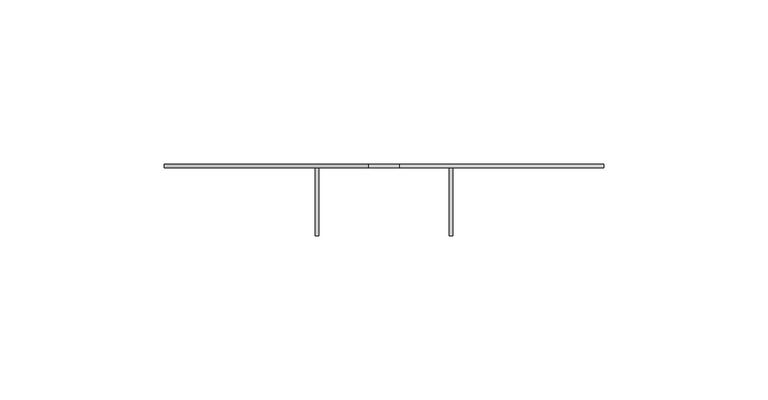
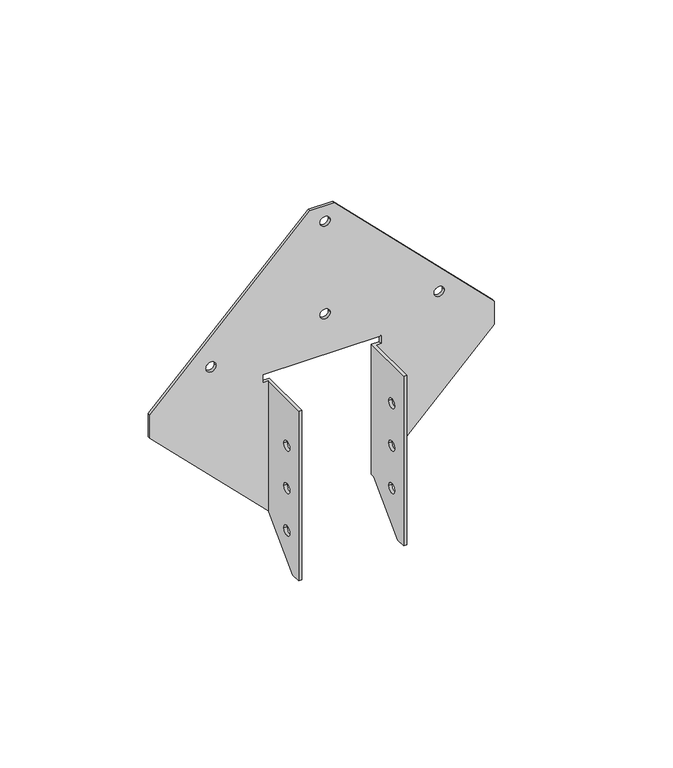
"""IFC4 building model written with IfcOpenShell, lengths in millimetres: proxy geometry, Simpson Strong-Tie H1 : Simpson Strong-Tie H1."""

from ifc_helpers import new_model, si_unit, frame, origin, place, context, project, spatial, polyline, circle_curve, source, transform, mapped, element, save
from ifc_brep_helpers import plane_surface, revolved_surface, advanced_brep


def generic_models_ac6e08b7(model_context):
    return source(origin(), model_context, "Body", "AdvancedBrep", [
        advanced_brep(
        [(-0.790575, 0.0, 54.76875), (-0.790575, -1.18872, 54.76875), (3.171825, -1.18872, 54.76875), (3.171825, 0.0, 54.76875), (-0.790575, 0.0, 16.66875), (-0.790575, -1.18872, 16.66875), (3.171825, -1.18872, 16.66875), (3.171825, 0.0, 16.66875), (43.659425, 0.0, 10.31875), (43.659425, -1.18872, 10.31875), (47.621825, -1.18872, 10.31875), (47.621825, 0.0, 10.31875), (-45.240575, 0.0, 10.31875), (-45.240575, -1.18872, 10.31875), (-41.278175, -1.18872, 10.31875), (-41.278175, 0.0, 10.31875), (19.84756, -11.902103, -19.05), (21.03628, -11.902103, -19.05), (21.03628, -15.864503, -19.05), (19.84756, -15.864503, -19.05), (19.84756, -11.902103, -36.5125), (21.03628, -11.902103, -36.5125), (21.03628, -15.864503, -36.5125), (19.84756, -15.864503, -36.5125), (19.84756, -11.902103, -53.975), (21.03628, -11.902103, -53.975), (21.03628, -15.864503, -53.975), (19.84756, -15.864503, -53.975), (-21.03628, -11.902103, -57.15), (-19.84756, -11.902103, -57.15), (-19.84756, -15.864503, -57.15), (-21.03628, -15.864503, -57.15), (-21.03628, -11.902103, -39.6875), (-19.84756, -11.902103, -39.6875), (-19.84756, -15.864503, -39.6875), (-21.03628, -15.864503, -39.6875), (-21.03628, -11.902103, -22.225), (-19.84756, -11.902103, -22.225), (-19.84756, -15.864503, -22.225), (-21.03628, -15.864503, -22.225), (23.08225, 0.0, 0.0), (23.08225, 0.0, -3.175), (23.08225, -1.18872, -3.175), (23.08225, -1.18872, 0.0), (21.03628, 0.0, -56.758894), (21.03628, -1.18872, -56.758894), (21.03628, -1.698923, -56.758894), (19.84756, -1.698923, -56.758894), (19.84756, 0.0, -56.758894), (19.84756, 0.0, -3.175), (19.84756, -21.820803, -3.175), (21.03628, -21.820803, -3.175), (21.03628, -1.18872, -3.175), (-23.08225, -1.18872, 0.0), (67.071875, -1.18872, -10.723299), (67.071875, -1.18872, -1.182951), (4.770174, -1.18872, 61.11875), (-4.770174, -1.18872, 61.11875), (-67.071875, -1.18872, -1.182951), (-67.071875, -1.18872, -10.723299), (-21.03628, -1.18872, -56.758894), (-21.03628, -1.18872, -3.175), (-23.08225, -1.18872, -3.175), (19.84756, -17.965029, -73.025), (19.84756, -21.820803, -73.025), (-21.03628, 0.0, -56.758894), (-19.84756, 0.0, -56.758894), (-19.84756, -1.698923, -56.758894), (-21.03628, -1.698923, -56.758894), (-23.08225, 0.0, 0.0), (-23.08225, 0.0, -3.175), (-19.84756, 0.0, -3.175), (-67.071875, 0.0, -10.723299), (-67.071875, 0.0, -1.182951), (-4.770174, 0.0, 61.11875), (4.770174, 0.0, 61.11875), (67.071875, 0.0, -1.182951), (67.071875, 0.0, -10.723299), (-21.03628, -21.820803, -3.175), (-19.84756, -21.820803, -3.175), (21.03628, -17.965029, -73.025), (21.03628, -21.820803, -73.025), (-19.84756, -21.820803, -73.025), (-19.84756, -17.965029, -73.025), (-21.03628, -17.965029, -73.025), (-21.03628, -21.820803, -73.025)],
        [
            (0, 1),
            (1, 2, circle_curve(frame((1.190625, -1.18872, 54.76875), z_axis=(0.0, -1.0, 0.0), x_axis=(-1.0, 0.0, 0.0)), 1.9812)),
            (2, 3),
            (3, 0, circle_curve(frame((1.190625, 0.0, 54.76875), z_axis=(0.0, 1.0, 0.0), x_axis=(-1.0, 0.0, 0.0)), 1.9812)),
            (4, 5),
            (5, 6, circle_curve(frame((1.190625, -1.18872, 16.66875), z_axis=(0.0, -1.0, 0.0), x_axis=(-1.0, 0.0, 0.0)), 1.9812)),
            (6, 7),
            (7, 4, circle_curve(frame((1.190625, 0.0, 16.66875), z_axis=(0.0, 1.0, 0.0), x_axis=(-1.0, 0.0, 0.0)), 1.9812)),
            (8, 9),
            (9, 10, circle_curve(frame((45.640625, -1.18872, 10.31875), z_axis=(0.0, -1.0, 0.0), x_axis=(-1.0, 0.0, 0.0)), 1.9812)),
            (10, 11),
            (11, 8, circle_curve(frame((45.640625, 0.0, 10.31875), z_axis=(0.0, 1.0, 0.0), x_axis=(-1.0, 0.0, 0.0)), 1.9812)),
            (12, 13),
            (13, 14, circle_curve(frame((-43.259375, -1.18872, 10.31875), z_axis=(0.0, -1.0, 0.0), x_axis=(-1.0, 0.0, 0.0)), 1.9812)),
            (14, 15),
            (15, 12, circle_curve(frame((-43.259375, 0.0, 10.31875), z_axis=(0.0, 1.0, 0.0), x_axis=(-1.0, 0.0, 0.0)), 1.9812)),
            (16, 17),
            (17, 18, circle_curve(frame((21.03628, -13.883303, -19.05), z_axis=(1.0, 0.0, 0.0), x_axis=(0.0, 1.0, 0.0)), 1.9812)),
            (18, 19),
            (19, 16, circle_curve(frame((19.84756, -13.883303, -19.05), z_axis=(-1.0, 0.0, 0.0), x_axis=(0.0, 1.0, 0.0)), 1.9812)),
            (20, 21),
            (21, 22, circle_curve(frame((21.03628, -13.883303, -36.5125), z_axis=(1.0, 0.0, 0.0), x_axis=(0.0, 1.0, 0.0)), 1.9812)),
            (22, 23),
            (23, 20, circle_curve(frame((19.84756, -13.883303, -36.5125), z_axis=(-1.0, 0.0, 0.0), x_axis=(0.0, 1.0, 0.0)), 1.9812)),
            (24, 25),
            (25, 26, circle_curve(frame((21.03628, -13.883303, -53.975), z_axis=(1.0, 0.0, 0.0), x_axis=(0.0, 1.0, 0.0)), 1.9812)),
            (26, 27),
            (27, 24, circle_curve(frame((19.84756, -13.883303, -53.975), z_axis=(-1.0, 0.0, 0.0), x_axis=(0.0, 1.0, 0.0)), 1.9812)),
            (28, 29),
            (29, 30, circle_curve(frame((-19.84756, -13.883303, -57.15), z_axis=(1.0, 0.0, 0.0), x_axis=(0.0, 1.0, 0.0)), 1.9812)),
            (30, 31),
            (31, 28, circle_curve(frame((-21.03628, -13.883303, -57.15), z_axis=(-1.0, 0.0, 0.0), x_axis=(0.0, 1.0, 0.0)), 1.9812)),
            (32, 33),
            (33, 34, circle_curve(frame((-19.84756, -13.883303, -39.6875), z_axis=(1.0, 0.0, 0.0), x_axis=(0.0, 1.0, 0.0)), 1.9812)),
            (34, 35),
            (35, 32, circle_curve(frame((-21.03628, -13.883303, -39.6875), z_axis=(-1.0, 0.0, 0.0), x_axis=(0.0, 1.0, 0.0)), 1.9812)),
            (36, 37),
            (37, 38, circle_curve(frame((-19.84756, -13.883303, -22.225), z_axis=(1.0, 0.0, 0.0), x_axis=(0.0, 1.0, 0.0)), 1.9812)),
            (38, 39),
            (39, 36, circle_curve(frame((-21.03628, -13.883303, -22.225), z_axis=(-1.0, 0.0, 0.0), x_axis=(0.0, 1.0, 0.0)), 1.9812)),
            (40, 41),
            (41, 42),
            (42, 43),
            (43, 40),
            (44, 45),
            (45, 46),
            (46, 47),
            (47, 48),
            (48, 44),
            (49, 50),
            (50, 51),
            (51, 52),
            (52, 42),
            (41, 49),
            (53, 43),
            (52, 45),
            (45, 54),
            (54, 55),
            (55, 56),
            (56, 57),
            (57, 58),
            (58, 59),
            (59, 60),
            (60, 61),
            (61, 62),
            (62, 53),
            (1, 2, circle_curve(frame((1.190625, -1.18872, 54.76875), z_axis=(0.0, 1.0, 0.0), x_axis=(-1.0, 0.0, 0.0)), 1.9812)),
            (5, 6, circle_curve(frame((1.190625, -1.18872, 16.66875), z_axis=(0.0, 1.0, 0.0), x_axis=(-1.0, 0.0, 0.0)), 1.9812)),
            (9, 10, circle_curve(frame((45.640625, -1.18872, 10.31875), z_axis=(0.0, 1.0, 0.0), x_axis=(-1.0, 0.0, 0.0)), 1.9812)),
            (13, 14, circle_curve(frame((-43.259375, -1.18872, 10.31875), z_axis=(0.0, 1.0, 0.0), x_axis=(-1.0, 0.0, 0.0)), 1.9812)),
            (47, 63),
            (63, 64),
            (64, 50),
            (49, 48),
            (19, 16, circle_curve(frame((19.84756, -13.883303, -19.05), z_axis=(1.0, 0.0, 0.0), x_axis=(0.0, 1.0, 0.0)), 1.9812)),
            (23, 20, circle_curve(frame((19.84756, -13.883303, -36.5125), z_axis=(1.0, 0.0, 0.0), x_axis=(0.0, 1.0, 0.0)), 1.9812)),
            (27, 24, circle_curve(frame((19.84756, -13.883303, -53.975), z_axis=(1.0, 0.0, 0.0), x_axis=(0.0, 1.0, 0.0)), 1.9812)),
            (60, 65),
            (65, 66),
            (66, 67),
            (67, 68),
            (68, 60),
            (40, 69),
            (69, 70),
            (70, 71),
            (71, 66),
            (65, 72),
            (72, 73),
            (73, 74),
            (74, 75),
            (75, 76),
            (76, 77),
            (77, 44),
            (3, 0, circle_curve(frame((1.190625, 0.0, 54.76875), z_axis=(0.0, -1.0, 0.0), x_axis=(-1.0, 0.0, 0.0)), 1.9812)),
            (7, 4, circle_curve(frame((1.190625, 0.0, 16.66875), z_axis=(0.0, -1.0, 0.0), x_axis=(-1.0, 0.0, 0.0)), 1.9812)),
            (11, 8, circle_curve(frame((45.640625, 0.0, 10.31875), z_axis=(0.0, -1.0, 0.0), x_axis=(-1.0, 0.0, 0.0)), 1.9812)),
            (15, 12, circle_curve(frame((-43.259375, 0.0, 10.31875), z_axis=(0.0, -1.0, 0.0), x_axis=(-1.0, 0.0, 0.0)), 1.9812)),
            (59, 72),
            (69, 53),
            (62, 70),
            (61, 78),
            (78, 79),
            (79, 71),
            (46, 80),
            (80, 63),
            (51, 81),
            (81, 80),
            (17, 18, circle_curve(frame((21.03628, -13.883303, -19.05), z_axis=(-1.0, 0.0, 0.0), x_axis=(0.0, 1.0, 0.0)), 1.9812)),
            (21, 22, circle_curve(frame((21.03628, -13.883303, -36.5125), z_axis=(-1.0, 0.0, 0.0), x_axis=(0.0, 1.0, 0.0)), 1.9812)),
            (25, 26, circle_curve(frame((21.03628, -13.883303, -53.975), z_axis=(-1.0, 0.0, 0.0), x_axis=(0.0, 1.0, 0.0)), 1.9812)),
            (79, 82),
            (82, 83),
            (83, 67),
            (29, 30, circle_curve(frame((-19.84756, -13.883303, -57.15), z_axis=(-1.0, 0.0, 0.0), x_axis=(0.0, 1.0, 0.0)), 1.9812)),
            (33, 34, circle_curve(frame((-19.84756, -13.883303, -39.6875), z_axis=(-1.0, 0.0, 0.0), x_axis=(0.0, 1.0, 0.0)), 1.9812)),
            (37, 38, circle_curve(frame((-19.84756, -13.883303, -22.225), z_axis=(-1.0, 0.0, 0.0), x_axis=(0.0, 1.0, 0.0)), 1.9812)),
            (68, 84),
            (84, 85),
            (85, 78),
            (31, 28, circle_curve(frame((-21.03628, -13.883303, -57.15), z_axis=(1.0, 0.0, 0.0), x_axis=(0.0, 1.0, 0.0)), 1.9812)),
            (35, 32, circle_curve(frame((-21.03628, -13.883303, -39.6875), z_axis=(1.0, 0.0, 0.0), x_axis=(0.0, 1.0, 0.0)), 1.9812)),
            (39, 36, circle_curve(frame((-21.03628, -13.883303, -22.225), z_axis=(1.0, 0.0, 0.0), x_axis=(0.0, 1.0, 0.0)), 1.9812)),
            (83, 84),
            (73, 58),
            (57, 74),
            (82, 85),
            (64, 81),
            (77, 54),
            (76, 55),
            (75, 56),
        ],
        [
            revolved_surface(polyline([(-0.790575, 0.0, 54.76875), (-0.790575, -1.18872, 54.76875)]), (1.190625, -1.18872, 54.76875), (0.0, 1.0, 0.0)),
            revolved_surface(polyline([(-0.790575, 0.0, 16.66875), (-0.790575, -1.18872, 16.66875)]), (1.190625, -1.18872, 16.66875), (0.0, 1.0, 0.0)),
            revolved_surface(polyline([(43.659425, 0.0, 10.31875), (43.659425, -1.18872, 10.31875)]), (45.640625, -1.18872, 10.31875), (0.0, 1.0, 0.0)),
            revolved_surface(polyline([(-45.240575, 0.0, 10.31875), (-45.240575, -1.18872, 10.31875)]), (-43.259375, -1.18872, 10.31875), (0.0, 1.0, 0.0)),
            revolved_surface(polyline([(19.84756, -11.902103, -19.05), (21.03628, -11.902103, -19.05)]), (21.03628, -13.883303, -19.05), (-1.0, 0.0, 0.0)),
            revolved_surface(polyline([(19.84756, -11.902103, -36.5125), (21.03628, -11.902103, -36.5125)]), (21.03628, -13.883303, -36.5125), (-1.0, 0.0, 0.0)),
            revolved_surface(polyline([(19.84756, -11.902103, -53.975), (21.03628, -11.902103, -53.975)]), (21.03628, -13.883303, -53.975), (-1.0, 0.0, 0.0)),
            revolved_surface(polyline([(-21.03628, -11.902103, -57.15), (-19.84756, -11.902103, -57.15)]), (-19.84756, -13.883303, -57.15), (-1.0, 0.0, 0.0)),
            revolved_surface(polyline([(-21.03628, -11.902103, -39.6875), (-19.84756, -11.902103, -39.6875)]), (-19.84756, -13.883303, -39.6875), (-1.0, 0.0, 0.0)),
            revolved_surface(polyline([(-21.03628, -11.902103, -22.225), (-19.84756, -11.902103, -22.225)]), (-19.84756, -13.883303, -22.225), (-1.0, 0.0, 0.0)),
            plane_surface(frame((23.08225, -1.18872, -3.175), z_axis=(-1.0, 0.0, 0.0), x_axis=(0.0, 0.0, 1.0))),
            plane_surface(frame((19.84756, 0.0, -56.758894), z_axis=(0.0, 0.0, -1.0), x_axis=(1.0, 0.0, 0.0))),
            plane_surface(frame((21.03628, -1.240453, -3.175), z_axis=(0.0, 0.0, 1.0), x_axis=(1.0, 0.0, 0.0))),
            plane_surface(frame((0.0, -1.18872, -12.3047323), z_axis=(0.0, -1.0, 0.0), x_axis=(1.0, 0.0, 0.0))),
            plane_surface(frame((19.84756, -22.735203, -12.3047323), z_axis=(-1.0, 0.0, 0.0), x_axis=(0.0, 1.0, 0.0))),
            plane_surface(frame((-19.84756, 0.0, -56.758894), z_axis=(0.0, 0.0, -1.0), x_axis=(-1.0, 0.0, 0.0))),
            plane_surface(frame((0.0, 0.0, -12.3047323), z_axis=(0.0, 1.0, 0.0), x_axis=(1.0, 0.0, 0.0))),
            plane_surface(frame((-67.071875, -1.18872, -10.723299), z_axis=(-0.7071067811865432, 0.0, -0.7071067811865518), x_axis=(0.0, 1.0, 0.0))),
            plane_surface(frame((-23.08225, -1.18872, -3.175), z_axis=(1.0, 0.0, 0.0), x_axis=(0.0, 0.0, 1.0))),
            plane_surface(frame((-21.03628, -21.820803, -3.175), z_axis=(0.0, 0.0, 1.0), x_axis=(-1.0, 0.0, 0.0))),
            plane_surface(frame((21.03628, -17.965029, -73.025), z_axis=(0.0, 0.7071067811865476, -0.7071067811865475), x_axis=(1.0, 0.0, 0.0))),
            plane_surface(frame((21.03628, -22.735203, -12.3047323), z_axis=(1.0, 0.0, 0.0), x_axis=(0.0, 1.0, 0.0))),
            plane_surface(frame((-19.84756, -22.735203, -12.3047323), z_axis=(1.0, 0.0, 0.0), x_axis=(0.0, -1.0, 0.0))),
            plane_surface(frame((-21.03628, -22.735203, -12.3047323), z_axis=(-1.0, 0.0, 0.0), x_axis=(0.0, -1.0, 0.0))),
            plane_surface(frame((-4.770174, -1.18872, 61.11875), z_axis=(-0.7071067811865518, 0.0, 0.7071067811865434), x_axis=(0.0, 1.0, 0.0))),
            plane_surface(frame((-67.071875, -1.18872, -1.182951), z_axis=(-1.0, 0.0, 0.0), x_axis=(0.0, 1.0, 0.0))),
            plane_surface(frame((-21.03628, -17.965029, -73.025), z_axis=(0.0, 0.0, -1.0), x_axis=(1.0, 0.0, 0.0))),
            plane_surface(frame((-21.03628, -21.820803, -73.025), z_axis=(0.0, -1.0, 0.0), x_axis=(-1.0, 0.0, 0.0))),
            plane_surface(frame((-21.49475, -1.18872, 0.0), z_axis=(0.0, 0.0, -1.0), x_axis=(0.0, 1.0, 0.0))),
            plane_surface(frame((21.03628, -21.820803, -3.175), z_axis=(0.0, -1.0, 0.0), x_axis=(-1.0, 0.0, 0.0))),
            plane_surface(frame((21.03628, -21.820803, -73.025), z_axis=(0.0, 0.0, -1.0), x_axis=(-1.0, 0.0, 0.0))),
            plane_surface(frame((4.770174, -1.18872, -73.025), z_axis=(0.7071067811865519, 0.0, -0.7071067811865431), x_axis=(0.0, -1.0, 0.0))),
            plane_surface(frame((67.071875, -1.18872, -10.723299), z_axis=(1.0, 0.0, 0.0), x_axis=(0.0, -1.0, 0.0))),
            plane_surface(frame((67.071875, -1.18872, -1.182951), z_axis=(0.707106781186543, 0.0, 0.707106781186552), x_axis=(0.0, -1.0, 0.0))),
            plane_surface(frame((4.770174, -1.18872, 61.11875), z_axis=(0.0, 0.0, 1.0), x_axis=(0.0, -1.0, 0.0))),
        ],
        [
            (0, [[1, 2, 3, 4]]),
            (1, [[5, 6, 7, 8]]),
            (2, [[9, 10, 11, 12]]),
            (3, [[13, 14, 15, 16]]),
            (4, [[17, 18, 19, 20]]),
            (5, [[21, 22, 23, 24]]),
            (6, [[25, 26, 27, 28]]),
            (7, [[29, 30, 31, 32]]),
            (8, [[33, 34, 35, 36]]),
            (9, [[37, 38, 39, 40]]),
            (10, [[41, 42, 43, 44]]),
            (11, [[45, 46, 47, 48, 49]]),
            (12, [[50, 51, 52, 53, -42, 54]]),
            (13, [[55, -43, -53, 56, 57, 58, 59, 60, 61, 62, 63, 64, 65, 66], [-2, 67], [-6, 68], [-10, 69], [-14, 70]]),
            (14, [[-48, 71, 72, 73, -50, 74], [75, -20], [76, -24], [77, -28]]),
            (15, [[78, 79, 80, 81, 82]]),
            (16, [[83, 84, 85, 86, -79, 87, 88, 89, 90, 91, 92, 93, -49, -74, -54, -41], [94, -4], [95, -8], [96, -12], [97, -16]]),
            (17, [[-78, -63, 98, -87]]),
            (18, [[-84, 99, -66, 100]]),
            (19, [[101, 102, 103, -85, -100, -65]]),
            (20, [[104, 105, -71, -47]]),
            (21, [[-56, -52, 106, 107, -104, -46], [-18, 108], [-22, 109], [-26, 110]]),
            (22, [[-80, -86, -103, 111, 112, 113], [-30, 114], [-34, 115], [-38, 116]]),
            (23, [[-82, 117, 118, 119, -101, -64], [120, -32], [121, -36], [122, -40]]),
            (9, [[-37, -122, -39, -116]]),
            (8, [[-33, -121, -35, -115]]),
            (7, [[-29, -120, -31, -114]]),
            (6, [[-25, -77, -27, -110]]),
            (5, [[-21, -76, -23, -109]]),
            (4, [[-17, -75, -19, -108]]),
            (20, [[-113, 123, -117, -81]]),
            (3, [[-13, -97, -15, -70]]),
            (2, [[-9, -96, -11, -69]]),
            (1, [[-5, -95, -7, -68]]),
            (0, [[-1, -94, -3, -67]]),
            (24, [[-89, 124, -61, 125]]),
            (25, [[-88, -98, -62, -124]]),
            (26, [[-112, 126, -118, -123]]),
            (27, [[-111, -102, -119, -126]]),
            (28, [[-55, -99, -83, -44]]),
            (29, [[-73, 127, -106, -51]]),
            (30, [[-72, -105, -107, -127]]),
            (31, [[-45, -93, 128, -57]]),
            (32, [[-92, 129, -58, -128]]),
            (33, [[-91, 130, -59, -129]]),
            (34, [[-90, -125, -60, -130]]),
        ],
    ),
    ])


if __name__ == "__main__":
    model = new_model("IFC4")
    model_context = context("Model", 3, world=origin())
    ifc_project = project(units=[si_unit("LENGTHUNIT", "METRE", prefix="MILLI")], contexts=[model_context])
    site = spatial("IfcSite", under=ifc_project)
    building = spatial("IfcBuilding", under=site)
    placement = place(None, origin())
    generic_models_shape = generic_models_ac6e08b7(model_context)
    element("IfcBuildingElementProxy", 1, Name="Simpson Strong-Tie H1 : Simpson Strong-Tie H1", ObjectType="Simpson Strong-Tie H1 : Simpson Strong-Tie H1", at=placement, inside=building, context=model_context, shape_type="MappedRepresentation", body=[
        mapped(generic_models_shape, transform((0.0, 0.0, 0.0), x_axis=(1.0, 0.0, 0.0), y_axis=(0.0, 1.0, 0.0), z_axis=(0.0, 0.0, 1.0))),
    ])
    save(model, "model.ifc")

# Revit data of these elements
# Type "Simpson Strong-Tie H1 : Simpson Strong-Tie H1"
#   Default Elevation = 0
# Element 1 (IfcBuildingElementProxy, "Simpson Strong-Tie H1 : Simpson Strong-Tie H1")
#   Materials on its faces: "Material __RGBA_0.749_0.749_0.749_1.000"
# Materials
#   "Material __RGBA_0.749_0.749_0.749_1.000": class "SAT", colour RGB 191 191 191, transparency 0
